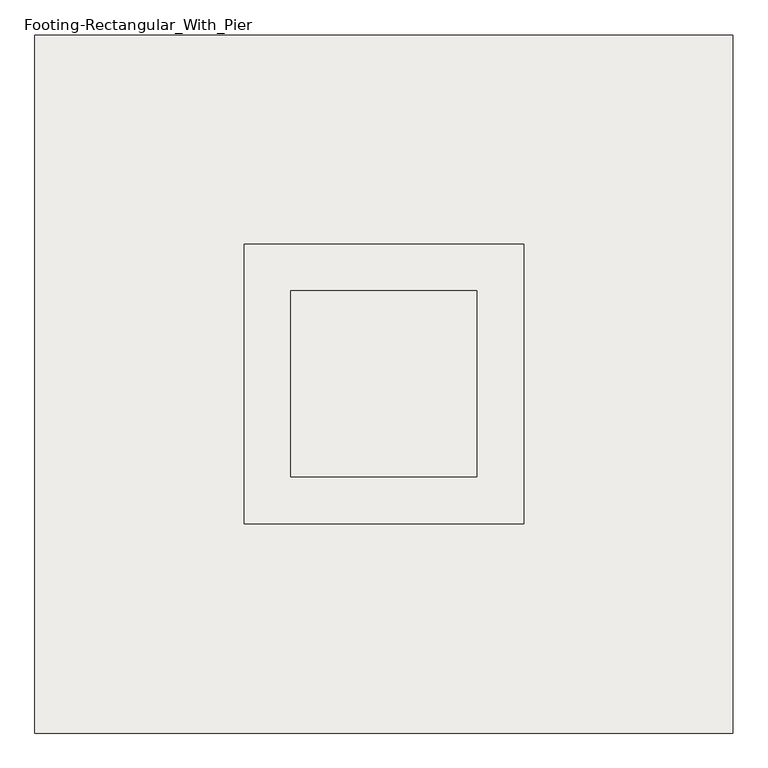
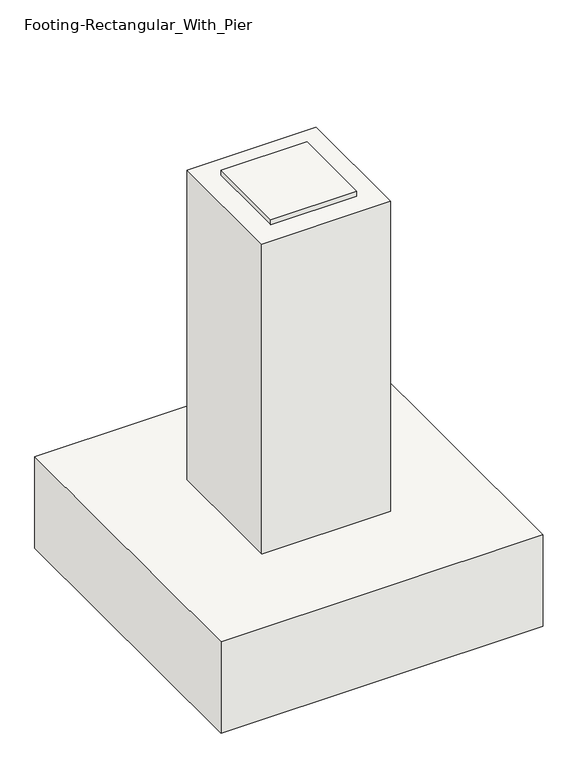
"""IFC4 building model written with IfcOpenShell, lengths in millimetres: slab geometry, Footing-Rectangular_With_Pier."""

from ifc_helpers import new_model, si_unit, frame, origin, origin_with_axes, place, context, project, spatial, polyline, outline, extrude, source, transform, mapped, element, save


def footing_rectangular_with_pier_95157401(model_context):
    return source(origin(), model_context, "Body", "SweptSolid", [
        extrude(outline(polyline([(203.2, 203.2), (203.2, -203.2), (-203.2, -203.2), (-203.2, 203.2), (203.2, 203.2)])), frame((0.0, 0.0, 1549.4), z_axis=(0.0, 0.0, 1.0), x_axis=(1.0, 0.0, 0.0)), (0.0, 0.0, 1.0), 25.4),
        extrude(outline(polyline([(762.0, 762.0), (762.0, -762.0), (-762.0, -762.0), (-762.0, 762.0), (762.0, 762.0)])), frame((0.0, 0.0, -457.2), z_axis=(0.0, 0.0, 1.0), x_axis=(1.0, 0.0, 0.0)), (0.0, 0.0, 1.0), 457.2),
        extrude(outline(polyline([(304.8, 304.8), (304.8, -304.8), (-304.8, -304.8), (-304.8, 304.8), (304.8, 304.8)])), origin_with_axes(), (0.0, 0.0, 1.0), 1549.4),
    ])


if __name__ == "__main__":
    model = new_model("IFC4")
    model_context = context("Model", 3, world=origin())
    ifc_project = project(units=[si_unit("LENGTHUNIT", "METRE", prefix="MILLI")], contexts=[model_context])
    site = spatial("IfcSite", under=ifc_project)
    building = spatial("IfcBuilding", under=site)
    placement = place(None, origin())
    footing_rectangular_with_pier_shape = footing_rectangular_with_pier_95157401(model_context)
    element("IfcSlab", 1, ObjectType="Footing-Rectangular_With_Pier : F8 - 5'-0\" x 5'-0\" x 1'-6\"", at=placement, inside=building, context=model_context, shape_type="MappedRepresentation", body=[
        mapped(footing_rectangular_with_pier_shape, transform((0.0, 0.0, 0.0), x_axis=(1.0, 0.0, 0.0), y_axis=(0.0, 1.0, 0.0), z_axis=(0.0, 0.0, 1.0))),
    ])
    save(model, "model.ifc")

# Revit data of these elements
# Type "Footing-Rectangular_With_Pier : F8 - 5'-0\" x 5'-0\" x 1'-6\""
#   Type Mark = "F8"
#   Assembly Code = "A1010100"
#   Width = 1524 mm
#   SteelPlateWidth [instance default] = 406.4 mm
#   SteelPlateThickness [instance default] = 25.4 mm
#   SteelPlateDepth [instance default] = 406.4 mm
#   PierWidth [instance default] = 609.6 mm
#   PierLength [instance default] = 609.6 mm
#   PierDepth [instance default] = 1371.6 mm
#   Length = 1524 mm
#   FootingThickness = 457.2 mm
#   Steel Plate = yes
#   Structural Material [instance default] = Concrete - Cast-in-Place Concrete
# Element 1 (IfcSlab, "Footing-Rectangular_With_Pier : F8 - 5'-0\" x 5'-0\" x 1'-6\"")
#   PierDepth = 1549.4 mm
#   Materials on its faces: "Concrete - Cast-in-Place Concrete", "Steel"
# Materials
#   "Concrete - Cast-in-Place Concrete": class "Concrete", colour RGB 192 192 192, transparency 0
#   "Steel": class "Metal", colour RGB 247 247 247, transparency 0, Description = "Steel, mill finish", Cost = 0
